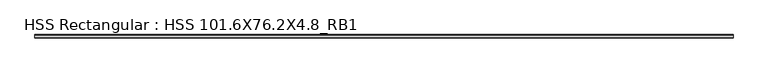
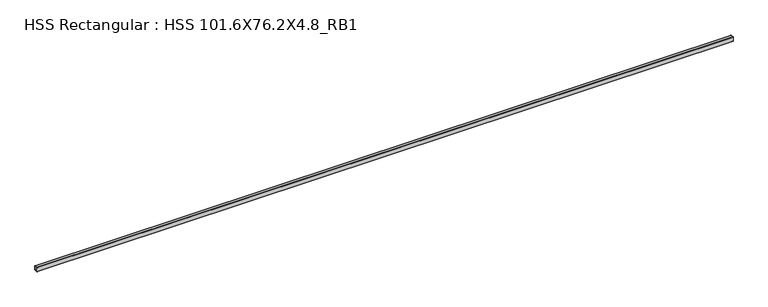
"""IFC4 building model written with IfcOpenShell, lengths in millimetres: beam geometry, HSS Rectangular : HSS 101.6X76.2X4.8_RB1."""

from ifc_helpers import new_model, si_unit, point, frame, frame_2d, origin, place, context, project, spatial, polyline, circle_curve, trimmed, segment, composite_curve, outline, extrude, source, transform, mapped, element, save


def hss_rectangular_hss_101_6x76_2x4_8_rb1_03b66c32(model_context):
    return source(origin(), model_context, "Body", "SweptSolid", [
        extrude(outline(composite_curve([segment(trimmed(circle_curve(frame_2d((-28.575, 41.275)), 9.525), [point((-38.1, 41.275))], [point((-28.575, 50.8))], False, "CARTESIAN"), True, "CONTINUOUS"), segment(polyline([(-28.575, 50.8), (28.575, 50.8)]), True, "CONTINUOUS"), segment(trimmed(circle_curve(frame_2d((28.575, 41.275)), 9.525), [point((28.575, 50.8))], [point((38.1, 41.275))], False, "CARTESIAN"), True, "CONTINUOUS"), segment(polyline([(38.1, 41.275), (38.1, -41.275)]), True, "CONTINUOUS"), segment(trimmed(circle_curve(frame_2d((28.575, -41.275)), 9.525), [point((38.1, -41.275))], [point((28.575, -50.8))], False, "CARTESIAN"), True, "CONTINUOUS"), segment(polyline([(28.575, -50.8), (-28.575, -50.8)]), True, "CONTINUOUS"), segment(trimmed(circle_curve(frame_2d((-28.575, -41.275)), 9.525), [point((-28.575, -50.8))], [point((-38.1, -41.275))], False, "CARTESIAN"), True, "CONTINUOUS"), segment(polyline([(-38.1, -41.275), (-38.1, 41.275)]), True, "CONTINUOUS")], self_intersect=False), holes=[composite_curve([segment(polyline([(28.575, 46.0375), (-28.575, 46.0375)]), True, "CONTINUOUS"), segment(trimmed(circle_curve(frame_2d((-28.575, 41.275)), 4.7625), [point((-28.575, 46.0375))], [point((-33.3375, 41.275))], True, "CARTESIAN"), True, "CONTINUOUS"), segment(polyline([(-33.3375, 41.275), (-33.3375, -41.275)]), True, "CONTINUOUS"), segment(trimmed(circle_curve(frame_2d((-28.575, -41.275)), 4.7625), [point((-33.3375, -41.275))], [point((-28.575, -46.0375))], True, "CARTESIAN"), True, "CONTINUOUS"), segment(polyline([(-28.575, -46.0375), (28.575, -46.0375)]), True, "CONTINUOUS"), segment(trimmed(circle_curve(frame_2d((28.575, -41.275)), 4.7625), [point((28.575, -46.0375))], [point((33.3375, -41.275))], True, "CARTESIAN"), True, "CONTINUOUS"), segment(polyline([(33.3375, -41.275), (33.3375, 41.275)]), True, "CONTINUOUS"), segment(trimmed(circle_curve(frame_2d((28.575, 41.275)), 4.7625), [point((33.3375, 41.275))], [point((28.575, 46.0375))], True, "CARTESIAN"), True, "CONTINUOUS")], self_intersect=False)]), frame((-8984.6643948, 0.0, 0.0), z_axis=(1.0, 0.0, 0.0), x_axis=(0.0, 1.0, 0.0)), (0.0, 0.0, 1.0), 14912.411789),
    ])


if __name__ == "__main__":
    model = new_model("IFC4")
    model_context = context("Model", 3, world=origin())
    ifc_project = project(units=[si_unit("LENGTHUNIT", "METRE", prefix="MILLI")], contexts=[model_context])
    site = spatial("IfcSite", under=ifc_project)
    building = spatial("IfcBuilding", under=site)
    placement = place(None, origin())
    hss_rectangular_hss_101_6x76_2x4_8_rb1_shape = hss_rectangular_hss_101_6x76_2x4_8_rb1_03b66c32(model_context)
    element("IfcBeam", 1, ObjectType="HSS Rectangular : HSS 101.6X76.2X4.8_RB1", at=placement, inside=building, context=model_context, shape_type="MappedRepresentation", body=[
        mapped(hss_rectangular_hss_101_6x76_2x4_8_rb1_shape, transform((0.0, 0.0, 0.0), x_axis=(1.0, 0.0, 0.0), y_axis=(0.0, 1.0, 0.0), z_axis=(0.0, 0.0, 1.0))),
    ])
    save(model, "model.ifc")

# Revit data of these elements
# Type "HSS Rectangular : HSS 101.6X76.2X4.8_RB1"
#   Section Name Key = "HSS 4X3X3/16"
#   Assembly Code = "B10"
#   Width = 7.62 cm
#   Wall Nominal Thickness = 0.4763 cm
#   Wall Design Thickness = 0.442 cm
#   Torsional Moment of Inertia = 260.561 cm⁴
#   Torsional Modulus = 61.2876 cm³
#   Section Area = 14.4516 cm²
#   Plastic Modulus weak axis = 40.3122 cm³
#   Plastic Modulus strong axis = 49.1612 cm³
#   Perimeter = 0.881482 m²/m
#   Outer Fillet = 0.9525 cm
#   Nominal Weight = 12.1285 kgf/m
#   Moment of Inertia weak axis = 131.529 cm⁴
#   Moment of Inertia strong axis = 205.202 cm⁴
#   Inner Fillet = 0.4763 cm
#   Height = 10.16 cm
#   Elastic Modulus weak axis = 34.4128 cm³
#   Elastic Modulus strong axis = 40.476 cm³
#   Centroid Vertical = 5.08 cm
#   Centroid Horizontal = 3.81 cm
#   Length [instance default] = 1524 mm
#   Structural Material [instance default] = Steel ASTM A500, Grade B, Rectangular and Square
#   Principal Axes Angle = 0
# Element 1 (IfcBeam, "HSS Rectangular : HSS 101.6X76.2X4.8_RB1")
#   Structural Material = Steel ASTM A992
#   Materials on its faces: "Steel ASTM A992"
# Materials
#   "Steel ASTM A500, Grade B, Rectangular and Square": class "Metal", colour RGB 199 199 199, transparency 0, Description = "Carbon steel", Cost = 0
#   "Steel ASTM A992": class "Metal", colour RGB 199 199 199, transparency 0, Description = "Structural steel 50ksi", Cost = 0
